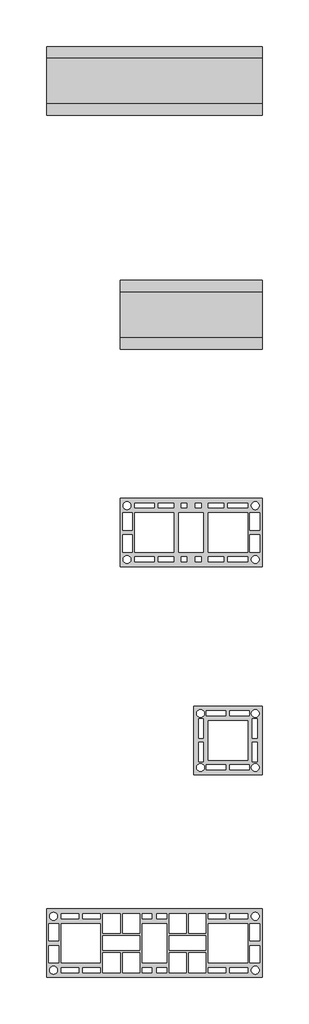
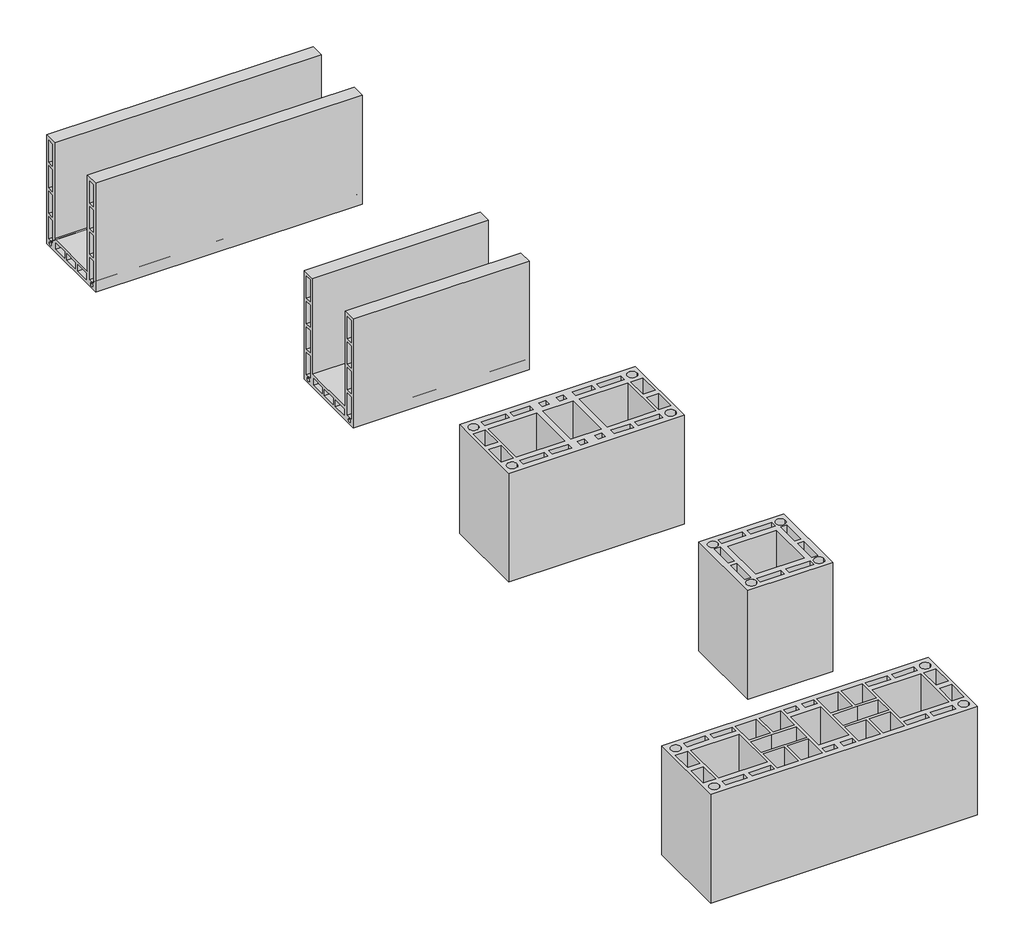
# One storey: 5 proxies.
"""IFC4 building model written with IfcOpenShell, lengths in millimetres."""

import ifcopenshell
import ifcopenshell.guid

model = None  # the IFC model being written
_history = None  # IfcOwnerHistory: only IFC2X3 demands one
_inside = {}  # id of a spatial element -> (the spatial element, [elements in it])
_under = {}  # id of a project, library or spatial element -> (it, [spatial elements below it])
_declared = {}  # id of a project -> (the project, [libraries it declares])
_typed = {}  # id of a type object -> (the type object, [elements of that type])
_made_of = {}  # id of a material, layer set ... -> (it, [elements and type objects made of it])


def new_model(schema):
    """Start an empty IFC model of exactly this schema.

    Asked for "IFC4X3", IfcOpenShell would pick the latest addendum, in which some entities
    have other attributes; the version numbers below select the first issue.
    IFC2X3 requires an IfcOwnerHistory on every rooted entity: one is made here for all.
    """
    global model, _history
    if schema == "IFC4X3":
        model = ifcopenshell.file(schema_version=(4, 3, 0, 0))
    else:
        model = ifcopenshell.file(schema=schema)
    _inside.clear()
    _under.clear()
    _declared.clear()
    _typed.clear()
    _made_of.clear()
    _history = None
    if model.schema == "IFC2X3":
        org = make("IfcOrganization", Name="unknown")
        user = make(
            "IfcPersonAndOrganization",
            ThePerson=make("IfcPerson", FamilyName="unknown"),
            TheOrganization=org,
        )
        app = make(
            "IfcApplication",
            ApplicationDeveloper=org,
            Version="unknown",
            ApplicationFullName="unknown",
            ApplicationIdentifier="unknown",
        )
        _history = make(
            "IfcOwnerHistory",
            OwningUser=user,
            OwningApplication=app,
            ChangeAction="ADDED",
            CreationDate=0,
        )
    return model


def make(cls, **values):
    """One entity of the class cls with the attributes given. An attribute that is None is left unset."""
    return model.create_entity(
        cls, **{name: value for name, value in values.items() if value is not None}
    )


def rooted(cls, **values):
    """An entity with a GlobalId (a new one), such as an element, a storey or a relation."""
    return make(cls, GlobalId=ifcopenshell.guid.new(), OwnerHistory=_history, **values)


def si_unit(unit_type, name, prefix=None):
    """IfcSIUnit, for example si_unit("LENGTHUNIT", "METRE", prefix="MILLI")."""
    return make("IfcSIUnit", UnitType=unit_type, Prefix=prefix, Name=name)


def assignment(units):
    """IfcUnitAssignment: the units of a project."""
    return None if units is None else make("IfcUnitAssignment", Units=units)


def point(xyz):
    """IfcCartesianPoint."""
    return None if xyz is None else make("IfcCartesianPoint", Coordinates=xyz)


def direction(xyz):
    """IfcDirection."""
    return None if xyz is None else make("IfcDirection", DirectionRatios=xyz)


def frame(location, z_axis=None, x_axis=None):
    """IfcAxis2Placement3D, a coordinate frame: its origin and axes. An axis left out is left unset."""
    return make(
        "IfcAxis2Placement3D",
        Location=point(location),
        Axis=direction(z_axis),
        RefDirection=direction(x_axis),
    )


def frame_2d(location, x_axis=None):
    """IfcAxis2Placement2D, a coordinate frame in the plane: its origin and x axis."""
    return make(
        "IfcAxis2Placement2D", Location=point(location), RefDirection=direction(x_axis)
    )


def origin():
    """The frame at (0, 0, 0) with its axes left unset."""
    return frame((0.0, 0.0, 0.0))


def origin_with_axes():
    """The frame at (0, 0, 0) with the z axis (0, 0, 1) and the x axis (1, 0, 0) written out."""
    return frame((0.0, 0.0, 0.0), z_axis=(0.0, 0.0, 1.0), x_axis=(1.0, 0.0, 0.0))


def place(relative_to, where):
    """IfcLocalPlacement: puts the frame where relative to a parent placement (None: the world)."""
    return make(
        "IfcLocalPlacement", PlacementRelTo=relative_to, RelativePlacement=where
    )


def context(
    kind, dimensions, precision=None, world=None, true_north=None, identifier=None
):
    """IfcGeometricRepresentationContext, for example the 3D "Model" context."""
    return make(
        "IfcGeometricRepresentationContext",
        ContextIdentifier=identifier,
        ContextType=kind,
        CoordinateSpaceDimension=dimensions,
        Precision=precision,
        WorldCoordinateSystem=world,
        TrueNorth=true_north,
    )


def project(units=None, contexts=None):
    """IfcProject with its units and contexts."""
    return rooted(
        "IfcProject",
        Name="project",
        RepresentationContexts=contexts,
        UnitsInContext=assignment(units),
    )


def spatial(cls, under=None, at=None, **own):
    """A site, building, storey or space (cls), placed at a placement, below another one or the project."""
    s = rooted(cls, ObjectPlacement=at, **own)
    if under is not None:
        _under.setdefault(under.id(), (under, []))[1].append(s)
    return s


def polyline(points):
    """IfcPolyline through the points."""
    return make("IfcPolyline", Points=[point(p) for p in points])


def circle_curve(where, radius):
    """IfcCircle in the frame where."""
    return make("IfcCircle", Position=where, Radius=radius)


def trimmed(basis, trim1, trim2, sense, master):
    """IfcTrimmedCurve: the piece of a basis curve between two trims."""
    return make(
        "IfcTrimmedCurve",
        BasisCurve=basis,
        Trim1=trim1,
        Trim2=trim2,
        SenseAgreement=sense,
        MasterRepresentation=master,
    )


def segment(curve, same_sense, transition):
    """IfcCompositeCurveSegment."""
    return make(
        "IfcCompositeCurveSegment",
        Transition=transition,
        SameSense=same_sense,
        ParentCurve=curve,
    )


def composite_curve(segments, self_intersect=None):
    """IfcCompositeCurve: segments joined end to end."""
    return make("IfcCompositeCurve", Segments=segments, SelfIntersect=self_intersect)


def outline(outer, holes=None, kind="AREA"):
    """IfcArbitraryClosedProfileDef: a profile drawn as a closed curve; with holes, ...WithVoids."""
    if holes is None:
        return make("IfcArbitraryClosedProfileDef", ProfileType=kind, OuterCurve=outer)
    return make(
        "IfcArbitraryProfileDefWithVoids",
        ProfileType=kind,
        OuterCurve=outer,
        InnerCurves=holes,
    )


def extrude(swept, where, along, depth):
    """IfcExtrudedAreaSolid: the profile swept, set in the frame where, extruded along a direction by depth."""
    return make(
        "IfcExtrudedAreaSolid",
        SweptArea=swept,
        Position=where,
        ExtrudedDirection=direction(along),
        Depth=depth,
    )


def shape(context_of_items, identifier, shape_type, items):
    """IfcShapeRepresentation: the items that make up one representation, for example the "Body"."""
    return make(
        "IfcShapeRepresentation",
        ContextOfItems=context_of_items,
        RepresentationIdentifier=identifier,
        RepresentationType=shape_type,
        Items=items,
    )


def source(mapping_origin, context_of_items, identifier, shape_type, items):
    """IfcRepresentationMap: a shape defined once, which mapped items show again and again."""
    return make(
        "IfcRepresentationMap",
        MappingOrigin=mapping_origin,
        MappedRepresentation=shape(context_of_items, identifier, shape_type, items),
    )


def transform(
    local_origin,
    x_axis=None,
    y_axis=None,
    z_axis=None,
    scale=None,
    scale2=None,
    scale3=None,
    uniform=True,
):
    """IfcCartesianTransformationOperator3D, or its non-uniform kind. x_axis, y_axis, z_axis: its Axis1, 2, 3."""
    if uniform:
        return make(
            "IfcCartesianTransformationOperator3D",
            Axis1=direction(x_axis),
            Axis2=direction(y_axis),
            LocalOrigin=point(local_origin),
            Scale=scale,
            Axis3=direction(z_axis),
        )
    return make(
        "IfcCartesianTransformationOperator3DnonUniform",
        Axis1=direction(x_axis),
        Axis2=direction(y_axis),
        LocalOrigin=point(local_origin),
        Scale=scale,
        Axis3=direction(z_axis),
        Scale2=scale2,
        Scale3=scale3,
    )


def mapped(mapping_source, mapping_target):
    """IfcMappedItem: shows the shape of a source again, moved by a transform."""
    return make(
        "IfcMappedItem", MappingSource=mapping_source, MappingTarget=mapping_target
    )


def made_of(thing, what):
    """Note that an element or type object is made of a material, layer set ...; save() writes the relation."""
    if what is not None:
        _made_of.setdefault(what.id(), (what, []))[1].append(thing)
    return thing


def element(
    cls,
    number,
    at=None,
    inside=None,
    cuts=None,
    type_object=None,
    material=None,
    context=None,
    identifier="Body",
    shape_type=None,
    held_by="IfcProductDefinitionShape",
    body=None,
    shapes=None,
    **own,
):
    """One element of the class cls, such as IfcWall. Its Tag is "e" and its number.

    at: its placement. inside: the storey or other place that contains it. cuts: it is an
    opening in that element (IfcRelVoidsElement). A single representation is given by context,
    identifier, shape_type and body (its items); several are given by shapes. held_by: the class
    of the entity that holds the representations. save() writes the other relations.
    """
    e = rooted(cls, Tag="e%d" % number, ObjectPlacement=at, **own)
    if body is not None:
        shapes = [shape(context, identifier, shape_type, body)]
    if shapes is not None:
        e.Representation = make(held_by, Representations=shapes)
    if inside is not None:
        _inside.setdefault(inside.id(), (inside, []))[1].append(e)
    if cuts is not None:
        rooted(
            "IfcRelVoidsElement", RelatingBuildingElement=cuts, RelatedOpeningElement=e
        )
    if type_object is not None:
        _typed.setdefault(type_object.id(), (type_object, []))[1].append(e)
    return made_of(e, material)


def aggregate(whole, parts):
    """IfcRelAggregates: a whole, such as a stair, and the parts it consists of."""
    return rooted("IfcRelAggregates", RelatingObject=whole, RelatedObjects=parts)


def save(model, path):
    """Write the relations noted so far, then the file.

    IfcRelAggregates (storeys below a building ...), IfcRelContainedInSpatialStructure (elements
    in a storey), IfcRelDefinesByType, IfcRelAssociatesMaterial and IfcRelDeclares: one each for
    every whole, place, type object, material and project.
    """
    for whole, parts in _under.values():
        aggregate(whole, parts)
    for where, things in _inside.values():
        rooted(
            "IfcRelContainedInSpatialStructure",
            RelatedElements=things,
            RelatingStructure=where,
        )
    for kind, things in _typed.values():
        rooted("IfcRelDefinesByType", RelatedObjects=things, RelatingType=kind)
    for what, things in _made_of.values():
        rooted("IfcRelAssociatesMaterial", RelatedObjects=things, RelatingMaterial=what)
    for by, libraries in _declared.values():
        rooted("IfcRelDeclares", RelatingContext=by, RelatedDefinitions=libraries)
    model.write(path)


def bloco_estrutural_de_15cm_l14_be15_329fd50e(model_context):
    return source(origin(), model_context, "Body", "SweptSolid", [
        extrude(outline(polyline([(0.0, 140.0), (140.0, 140.0), (140.0, 0.0), (0.0, 0.0), (0.0, 140.0)]), holes=[polyline([(30.0, 110.0), (30.0, 30.0), (110.0, 30.0), (110.0, 110.0), (30.0, 110.0)]), composite_curve([segment(trimmed(circle_curve(frame_2d((14.1087523, 124.7509514)), 8.0), [point((6.1087523, 124.7509514))], [point((22.1087523, 124.7509514))], True, "CARTESIAN"), True, "CONTINUOUS"), segment(trimmed(circle_curve(frame_2d((14.1087523, 124.7509514)), 8.0), [point((22.1087523, 124.7509514))], [point((6.1087523, 124.7509514))], True, "CARTESIAN"), True, "CONTINUOUS")], self_intersect=False), composite_curve([segment(trimmed(circle_curve(frame_2d((14.1087523, 14.7509514)), 8.0), [point((6.1087523, 14.7509514))], [point((22.1087523, 14.7509514))], True, "CARTESIAN"), True, "CONTINUOUS"), segment(trimmed(circle_curve(frame_2d((14.1087523, 14.7509514)), 8.0), [point((22.1087523, 14.7509514))], [point((6.1087523, 14.7509514))], True, "CARTESIAN"), True, "CONTINUOUS")], self_intersect=False), polyline([(20.0, 66.0), (10.0, 66.0), (10.0, 26.0), (20.0, 26.0), (20.0, 66.0)]), polyline([(20.0, 74.0), (20.0, 114.0), (10.0, 114.0), (10.0, 74.0), (20.0, 74.0)]), composite_curve([segment(trimmed(circle_curve(frame_2d((125.8912477, 124.7509514)), 8.0), [point((133.8912477, 124.7509514))], [point((117.8912477, 124.7509514))], True, "CARTESIAN"), True, "CONTINUOUS"), segment(trimmed(circle_curve(frame_2d((125.8912477, 124.7509514)), 8.0), [point((117.8912477, 124.7509514))], [point((133.8912477, 124.7509514))], True, "CARTESIAN"), True, "CONTINUOUS")], self_intersect=False), composite_curve([segment(trimmed(circle_curve(frame_2d((125.8912477, 14.7509514)), 8.0), [point((133.8912477, 14.7509514))], [point((117.8912477, 14.7509514))], True, "CARTESIAN"), True, "CONTINUOUS"), segment(trimmed(circle_curve(frame_2d((125.8912477, 14.7509514)), 8.0), [point((117.8912477, 14.7509514))], [point((133.8912477, 14.7509514))], True, "CARTESIAN"), True, "CONTINUOUS")], self_intersect=False), polyline([(120.0, 66.0), (120.0, 26.0), (130.0, 26.0), (130.0, 66.0), (120.0, 66.0)]), polyline([(120.0, 74.0), (130.0, 74.0), (130.0, 114.0), (120.0, 114.0), (120.0, 74.0)]), polyline([(66.0, 120.0), (66.0, 130.0), (26.0, 130.0), (26.0, 120.0), (66.0, 120.0)]), polyline([(74.0, 120.0), (114.0, 120.0), (114.0, 130.0), (74.0, 130.0), (74.0, 120.0)]), polyline([(66.0, 20.0), (26.0, 20.0), (26.0, 10.0), (66.0, 10.0), (66.0, 20.0)]), polyline([(74.0, 20.0), (74.0, 10.0), (114.0, 10.0), (114.0, 20.0), (74.0, 20.0)])]), origin_with_axes(), (0.0, 0.0, 1.0), 190.0),
    ])


def bloco_estrutural_de_30cm_l14_be30_19b25b02(model_context):
    return source(origin(), model_context, "Body", "SweptSolid", [
        extrude(outline(polyline([(290.0, 0.0), (0.0, 0.0), (0.0, 140.0), (290.0, 140.0), (290.0, 0.0)]), holes=[composite_curve([segment(trimmed(circle_curve(frame_2d((14.1087523, 124.7509514)), 8.0), [point((6.1087523, 124.7509514))], [point((22.1087523, 124.7509514))], True, "CARTESIAN"), True, "CONTINUOUS"), segment(trimmed(circle_curve(frame_2d((14.1087523, 124.7509514)), 8.0), [point((22.1087523, 124.7509514))], [point((6.1087523, 124.7509514))], True, "CARTESIAN"), True, "CONTINUOUS")], self_intersect=False), composite_curve([segment(trimmed(circle_curve(frame_2d((14.1087523, 14.7509514)), 8.0), [point((6.1087523, 14.7509514))], [point((22.1087523, 14.7509514))], True, "CARTESIAN"), True, "CONTINUOUS"), segment(trimmed(circle_curve(frame_2d((14.1087523, 14.7509514)), 8.0), [point((22.1087523, 14.7509514))], [point((6.1087523, 14.7509514))], True, "CARTESIAN"), True, "CONTINUOUS")], self_intersect=False), polyline([(110.0, 110.0), (30.0, 110.0), (30.0, 30.0), (110.0, 30.0), (110.0, 110.0)]), polyline([(170.0, 110.0), (120.0, 110.0), (120.0, 30.0), (170.0, 30.0), (170.0, 110.0)]), polyline([(70.0, 130.0), (30.0, 130.0), (30.0, 120.0), (70.0, 120.0), (70.0, 130.0)]), polyline([(70.0, 20.0), (30.0, 20.0), (30.0, 10.0), (70.0, 10.0), (70.0, 20.0)]), polyline([(78.0, 130.0), (78.0, 120.0), (110.0, 120.0), (110.0, 130.0), (78.0, 130.0)]), polyline([(78.0, 20.0), (78.0, 10.0), (110.0, 10.0), (110.0, 20.0), (78.0, 20.0)]), composite_curve([segment(trimmed(circle_curve(frame_2d((275.8912477, 124.7509514)), 8.0), [point((283.8912477, 124.7509514))], [point((267.8912477, 124.7509514))], True, "CARTESIAN"), True, "CONTINUOUS"), segment(trimmed(circle_curve(frame_2d((275.8912477, 124.7509514)), 8.0), [point((267.8912477, 124.7509514))], [point((283.8912477, 124.7509514))], True, "CARTESIAN"), True, "CONTINUOUS")], self_intersect=False), composite_curve([segment(trimmed(circle_curve(frame_2d((275.8912477, 14.7509514)), 8.0), [point((283.8912477, 14.7509514))], [point((267.8912477, 14.7509514))], True, "CARTESIAN"), True, "CONTINUOUS"), segment(trimmed(circle_curve(frame_2d((275.8912477, 14.7509514)), 8.0), [point((267.8912477, 14.7509514))], [point((283.8912477, 14.7509514))], True, "CARTESIAN"), True, "CONTINUOUS")], self_intersect=False), polyline([(180.0, 110.0), (180.0, 30.0), (260.0, 30.0), (260.0, 110.0), (180.0, 110.0)]), polyline([(220.0, 130.0), (220.0, 120.0), (260.0, 120.0), (260.0, 130.0), (220.0, 130.0)]), polyline([(220.0, 20.0), (220.0, 10.0), (260.0, 10.0), (260.0, 20.0), (220.0, 20.0)]), polyline([(212.0, 130.0), (180.0, 130.0), (180.0, 120.0), (212.0, 120.0), (212.0, 130.0)]), polyline([(212.0, 20.0), (180.0, 20.0), (180.0, 10.0), (212.0, 10.0), (212.0, 20.0)]), polyline([(25.0, 110.0), (5.0, 110.0), (5.0, 75.0), (25.0, 75.0), (25.0, 110.0)]), polyline([(25.0, 30.0), (25.0, 65.0), (5.0, 65.0), (5.0, 30.0), (25.0, 30.0)]), polyline([(265.0, 110.0), (265.0, 75.0), (285.0, 75.0), (285.0, 110.0), (265.0, 110.0)]), polyline([(265.0, 30.0), (285.0, 30.0), (285.0, 65.0), (265.0, 65.0), (265.0, 30.0)]), polyline([(153.5, 20.0), (153.5, 10.0), (165.5, 10.0), (165.5, 20.0), (153.5, 20.0)]), polyline([(136.5, 20.0), (124.5, 20.0), (124.5, 10.0), (136.5, 10.0), (136.5, 20.0)]), polyline([(153.5, 120.0), (165.5, 120.0), (165.5, 130.0), (153.5, 130.0), (153.5, 120.0)]), polyline([(136.5, 120.0), (136.5, 130.0), (124.5, 130.0), (124.5, 120.0), (136.5, 120.0)])]), origin_with_axes(), (0.0, 0.0, 1.0), 190.0),
    ])


def bloco_estrutural_de_45cm_l14_be45_067f568e(model_context):
    return source(origin(), model_context, "Body", "SweptSolid", [
        extrude(outline(polyline([(440.0, 0.0), (0.0, 0.0), (0.0, 140.0), (440.0, 140.0), (440.0, 0.0)]), holes=[composite_curve([segment(trimmed(circle_curve(frame_2d((14.1087523, 124.7509514)), 8.0), [point((6.1087523, 124.7509514))], [point((22.1087523, 124.7509514))], True, "CARTESIAN"), True, "CONTINUOUS"), segment(trimmed(circle_curve(frame_2d((14.1087523, 124.7509514)), 8.0), [point((22.1087523, 124.7509514))], [point((6.1087523, 124.7509514))], True, "CARTESIAN"), True, "CONTINUOUS")], self_intersect=False), composite_curve([segment(trimmed(circle_curve(frame_2d((14.1087523, 14.7509514)), 8.0), [point((6.1087523, 14.7509514))], [point((22.1087523, 14.7509514))], True, "CARTESIAN"), True, "CONTINUOUS"), segment(trimmed(circle_curve(frame_2d((14.1087523, 14.7509514)), 8.0), [point((22.1087523, 14.7509514))], [point((6.1087523, 14.7509514))], True, "CARTESIAN"), True, "CONTINUOUS")], self_intersect=False), polyline([(110.0, 110.0), (30.0, 110.0), (30.0, 30.0), (110.0, 30.0), (110.0, 110.0)]), polyline([(245.0, 110.0), (195.0, 110.0), (195.0, 30.0), (245.0, 30.0), (245.0, 110.0)]), polyline([(66.0, 130.0), (30.0, 130.0), (30.0, 120.0), (66.0, 120.0), (66.0, 130.0)]), polyline([(66.0, 20.0), (30.0, 20.0), (30.0, 10.0), (66.0, 10.0), (66.0, 20.0)]), polyline([(74.0, 130.0), (74.0, 120.0), (110.0, 120.0), (110.0, 130.0), (74.0, 130.0)]), polyline([(74.0, 20.0), (74.0, 10.0), (110.0, 10.0), (110.0, 20.0), (74.0, 20.0)]), composite_curve([segment(trimmed(circle_curve(frame_2d((425.8912477, 124.7509514)), 8.0), [point((433.8912477, 124.7509514))], [point((417.8912477, 124.7509514))], True, "CARTESIAN"), True, "CONTINUOUS"), segment(trimmed(circle_curve(frame_2d((425.8912477, 124.7509514)), 8.0), [point((417.8912477, 124.7509514))], [point((433.8912477, 124.7509514))], True, "CARTESIAN"), True, "CONTINUOUS")], self_intersect=False), composite_curve([segment(trimmed(circle_curve(frame_2d((425.8912477, 14.7509514)), 8.0), [point((433.8912477, 14.7509514))], [point((417.8912477, 14.7509514))], True, "CARTESIAN"), True, "CONTINUOUS"), segment(trimmed(circle_curve(frame_2d((425.8912477, 14.7509514)), 8.0), [point((417.8912477, 14.7509514))], [point((433.8912477, 14.7509514))], True, "CARTESIAN"), True, "CONTINUOUS")], self_intersect=False), polyline([(330.0, 110.0), (330.0, 30.0), (410.0, 30.0), (410.0, 110.0), (330.0, 110.0)]), polyline([(374.0, 130.0), (374.0, 120.0), (410.0, 120.0), (410.0, 130.0), (374.0, 130.0)]), polyline([(374.0, 20.0), (374.0, 10.0), (410.0, 10.0), (410.0, 20.0), (374.0, 20.0)]), polyline([(366.0, 130.0), (330.0, 130.0), (330.0, 120.0), (366.0, 120.0), (366.0, 130.0)]), polyline([(366.0, 20.0), (330.0, 20.0), (330.0, 10.0), (366.0, 10.0), (366.0, 20.0)]), polyline([(25.0, 110.0), (5.0, 110.0), (5.0, 75.0), (25.0, 75.0), (25.0, 110.0)]), polyline([(25.0, 30.0), (25.0, 65.0), (5.0, 65.0), (5.0, 30.0), (25.0, 30.0)]), polyline([(415.0, 110.0), (415.0, 75.0), (435.0, 75.0), (435.0, 110.0), (415.0, 110.0)]), polyline([(415.0, 30.0), (435.0, 30.0), (435.0, 65.0), (415.0, 65.0), (415.0, 30.0)]), polyline([(225.0, 20.0), (225.0, 10.0), (245.0, 10.0), (245.0, 20.0), (225.0, 20.0)]), polyline([(215.0, 20.0), (195.0, 20.0), (195.0, 10.0), (215.0, 10.0), (215.0, 20.0)]), polyline([(225.0, 120.0), (245.0, 120.0), (245.0, 130.0), (225.0, 130.0), (225.0, 120.0)]), polyline([(215.0, 120.0), (215.0, 130.0), (195.0, 130.0), (195.0, 120.0), (215.0, 120.0)]), polyline([(150.0, 130.0), (115.0, 130.0), (115.0, 90.0), (150.0, 90.0), (150.0, 130.0)]), polyline([(190.0, 130.0), (155.0, 130.0), (155.0, 90.0), (190.0, 90.0), (190.0, 130.0)]), polyline([(115.0, 85.0), (115.0, 55.0), (190.0, 55.0), (190.0, 85.0), (148.9828076, 85.0), (115.0, 85.0)]), polyline([(155.0, 50.0), (155.0, 10.0), (190.0, 10.0), (190.0, 50.0), (155.0, 50.0)]), polyline([(150.0, 10.0), (150.0, 50.0), (115.0, 50.0), (115.0, 10.0), (150.0, 10.0)]), polyline([(290.0, 130.0), (290.0, 90.0), (325.0, 90.0), (325.0, 130.0), (290.0, 130.0)]), polyline([(250.0, 130.0), (250.0, 90.0), (285.0, 90.0), (285.0, 130.0), (250.0, 130.0)]), polyline([(325.0, 85.0), (291.0171924, 85.0), (250.0, 85.0), (250.0, 55.0), (291.0171924, 55.0), (325.0, 55.0), (325.0, 85.0)]), polyline([(285.0, 50.0), (250.0, 50.0), (250.0, 10.0), (285.0, 10.0), (285.0, 50.0)]), polyline([(290.0, 10.0), (325.0, 10.0), (325.0, 50.0), (290.0, 50.0), (290.0, 10.0)])]), origin_with_axes(), (0.0, 0.0, 1.0), 190.0),
    ])


def canaleta_l14_c30_6f9dc855(model_context):
    return source(origin(), model_context, "Body", "SweptSolid", [
        extrude(outline(polyline([(140.0, 0.0), (0.0, 0.0), (0.0, 190.0), (23.0, 190.0), (23.0, 23.0), (117.0, 23.0), (117.0, 190.0), (140.0, 190.0), (140.0, 0.0)]), holes=[polyline([(123.0, 184.0), (123.0, 145.5), (134.0, 145.5), (134.0, 184.0), (123.0, 184.0)]), polyline([(123.0, 139.5), (123.0, 101.0), (134.0, 101.0), (134.0, 139.5), (123.0, 139.5)]), polyline([(123.0, 95.0), (123.0, 56.5), (134.0, 56.5), (134.0, 95.0), (123.0, 95.0)]), polyline([(123.0, 50.5), (123.0, 12.0), (134.0, 12.0), (134.0, 50.5), (123.0, 50.5)]), composite_curve([segment(trimmed(circle_curve(frame_2d((128.9426557, 6.2112346)), 3.0), [point((125.9426557, 6.2112346))], [point((131.9426557, 6.2112346))], True, "CARTESIAN"), True, "CONTINUOUS"), segment(trimmed(circle_curve(frame_2d((128.9426557, 6.2112346)), 3.0), [point((131.9426557, 6.2112346))], [point((125.9426557, 6.2112346))], True, "CARTESIAN"), True, "CONTINUOUS")], self_intersect=False), polyline([(17.0, 184.0), (6.0, 184.0), (6.0, 145.5), (17.0, 145.5), (17.0, 184.0)]), polyline([(17.0, 139.5), (6.0, 139.5), (6.0, 101.0), (17.0, 101.0), (17.0, 139.5)]), polyline([(17.0, 95.0), (6.0, 95.0), (6.0, 56.5), (17.0, 56.5), (17.0, 95.0)]), polyline([(17.0, 50.5), (6.0, 50.5), (6.0, 12.0), (17.0, 12.0), (17.0, 50.5)]), composite_curve([segment(trimmed(circle_curve(frame_2d((11.0573443, 6.2112346)), 3.0), [point((8.0573443, 6.2112346))], [point((14.0573443, 6.2112346))], True, "CARTESIAN"), True, "CONTINUOUS"), segment(trimmed(circle_curve(frame_2d((11.0573443, 6.2112346)), 3.0), [point((14.0573443, 6.2112346))], [point((8.0573443, 6.2112346))], True, "CARTESIAN"), True, "CONTINUOUS")], self_intersect=False), polyline([(88.5, 17.0), (88.5, 6.0), (113.5, 6.0), (113.5, 17.0), (88.5, 17.0)]), polyline([(57.5, 17.0), (57.5, 6.0), (82.5, 6.0), (82.5, 17.0), (57.5, 17.0)]), polyline([(26.5, 17.0), (26.5, 6.0), (51.5, 6.0), (51.5, 17.0), (26.5, 17.0)])]), frame((0.0, 0.0, 0.0), z_axis=(1.0, 0.0, 0.0), x_axis=(0.0, 1.0, 0.0)), (0.0, 0.0, 1.0), 290.0),
    ])


def canaleta_l14_c45_c2fd00c5(model_context):
    return source(origin(), model_context, "Body", "SweptSolid", [
        extrude(outline(polyline([(140.0, 0.0), (0.0, 0.0), (0.0, 190.0), (23.0, 190.0), (23.0, 23.0), (117.0, 23.0), (117.0, 190.0), (140.0, 190.0), (140.0, 0.0)]), holes=[polyline([(123.0, 184.0), (123.0, 145.5), (134.0, 145.5), (134.0, 184.0), (123.0, 184.0)]), polyline([(123.0, 139.5), (123.0, 101.0), (134.0, 101.0), (134.0, 139.5), (123.0, 139.5)]), polyline([(123.0, 95.0), (123.0, 56.5), (134.0, 56.5), (134.0, 95.0), (123.0, 95.0)]), polyline([(123.0, 50.5), (123.0, 12.0), (134.0, 12.0), (134.0, 50.5), (123.0, 50.5)]), composite_curve([segment(trimmed(circle_curve(frame_2d((128.9426557, 6.2112346)), 3.0), [point((125.9426557, 6.2112346))], [point((131.9426557, 6.2112346))], True, "CARTESIAN"), True, "CONTINUOUS"), segment(trimmed(circle_curve(frame_2d((128.9426557, 6.2112346)), 3.0), [point((131.9426557, 6.2112346))], [point((125.9426557, 6.2112346))], True, "CARTESIAN"), True, "CONTINUOUS")], self_intersect=False), polyline([(17.0, 184.0), (6.0, 184.0), (6.0, 145.5), (17.0, 145.5), (17.0, 184.0)]), polyline([(17.0, 139.5), (6.0, 139.5), (6.0, 101.0), (17.0, 101.0), (17.0, 139.5)]), polyline([(17.0, 95.0), (6.0, 95.0), (6.0, 56.5), (17.0, 56.5), (17.0, 95.0)]), polyline([(17.0, 50.5), (6.0, 50.5), (6.0, 12.0), (17.0, 12.0), (17.0, 50.5)]), composite_curve([segment(trimmed(circle_curve(frame_2d((11.0573443, 6.2112346)), 3.0), [point((8.0573443, 6.2112346))], [point((14.0573443, 6.2112346))], True, "CARTESIAN"), True, "CONTINUOUS"), segment(trimmed(circle_curve(frame_2d((11.0573443, 6.2112346)), 3.0), [point((14.0573443, 6.2112346))], [point((8.0573443, 6.2112346))], True, "CARTESIAN"), True, "CONTINUOUS")], self_intersect=False), polyline([(88.5, 17.0), (88.5, 6.0), (113.5, 6.0), (113.5, 17.0), (88.5, 17.0)]), polyline([(57.5, 17.0), (57.5, 6.0), (82.5, 6.0), (82.5, 17.0), (57.5, 17.0)]), polyline([(26.5, 17.0), (26.5, 6.0), (51.5, 6.0), (51.5, 17.0), (26.5, 17.0)])]), frame((0.0, 0.0, 0.0), z_axis=(1.0, 0.0, 0.0), x_axis=(0.0, 1.0, 0.0)), (0.0, 0.0, 1.0), 440.0),
    ])


model = new_model("IFC4")

# Units and contexts
model_context = context("Model", 3, world=origin())
ifc_project = project(units=[si_unit("LENGTHUNIT", "METRE", prefix="MILLI")], contexts=[model_context])

# Site, building, storey
site = spatial("IfcSite", under=ifc_project)
building = spatial("IfcBuilding", under=site)
storey = spatial("IfcBuildingStorey", under=building, Name="Nível 1", Elevation=0.0)

# Proxies
placement = place(None, origin())
bloco_estrutural_de_15cm_l14_be15_shape = bloco_estrutural_de_15cm_l14_be15_329fd50e(model_context)
element("IfcBuildingElementProxy", 1, Name="Bloco Estrutural de 15cm (L14) : BE15", ObjectType="Bloco Estrutural de 15cm (L14) : BE15", at=placement, inside=storey, context=model_context, shape_type="MappedRepresentation", body=[
    mapped(bloco_estrutural_de_15cm_l14_be15_shape, transform((2691.9297154, 1590.0313854, 0.0), x_axis=(1.0, 0.0, 0.0), y_axis=(0.0, 1.0, 0.0), z_axis=(0.0, 0.0, 1.0))),
])
bloco_estrutural_de_30cm_l14_be30_shape = bloco_estrutural_de_30cm_l14_be30_19b25b02(model_context)
element("IfcBuildingElementProxy", 2, Name="Bloco Estrutural de 30cm (L14) : BE30", ObjectType="Bloco Estrutural de 30cm (L14) : BE30", at=placement, inside=storey, context=model_context, shape_type="MappedRepresentation", body=[
    mapped(bloco_estrutural_de_30cm_l14_be30_shape, transform((2541.9297154, 2014.2243668, 0.0), x_axis=(1.0, 0.0, 0.0), y_axis=(0.0, 1.0, 0.0), z_axis=(0.0, 0.0, 1.0))),
])
bloco_estrutural_de_45cm_l14_be45_shape = bloco_estrutural_de_45cm_l14_be45_067f568e(model_context)
element("IfcBuildingElementProxy", 3, Name="Bloco Estrutural de 45cm (L14) : BE45", ObjectType="Bloco Estrutural de 45cm (L14) : BE45", at=placement, inside=storey, context=model_context, shape_type="MappedRepresentation", body=[
    mapped(bloco_estrutural_de_45cm_l14_be45_shape, transform((2391.9297154, 1176.4687225, 0.0), x_axis=(1.0, 0.0, 0.0), y_axis=(0.0, 1.0, 0.0), z_axis=(0.0, 0.0, 1.0))),
])
canaleta_l14_c30_shape = canaleta_l14_c30_6f9dc855(model_context)
element("IfcBuildingElementProxy", 4, Name="Canaleta (L14) : C30", ObjectType="Canaleta (L14) : C30", at=placement, inside=storey, context=model_context, shape_type="MappedRepresentation", body=[
    mapped(canaleta_l14_c30_shape, transform((2541.9297154, 2458.4083893, 0.0), x_axis=(1.0, 0.0, 0.0), y_axis=(0.0, 1.0, 0.0), z_axis=(0.0, 0.0, 1.0))),
])
canaleta_l14_c45_shape = canaleta_l14_c45_c2fd00c5(model_context)
element("IfcBuildingElementProxy", 5, Name="Canaleta (L14) : C45", ObjectType="Canaleta (L14) : C45", at=placement, inside=storey, context=model_context, shape_type="MappedRepresentation", body=[
    mapped(canaleta_l14_c45_shape, transform((2391.9297154, 2935.4953738, 0.0), x_axis=(1.0, 0.0, 0.0), y_axis=(0.0, 1.0, 0.0), z_axis=(0.0, 0.0, 1.0))),
])

save(model, "model.ifc")

# Revit data of these elements
# Project information
#   Data de emissão do projeto = "Data de emissão"
#   Status do projeto = "Status do projeto"
#   Nome do cliente = "Proprietário"
#   Endereço do projeto = "Enter address here"
#   Nome do projeto = "Nome do projeto"
#   Número do projeto = "0001"
# Type "Bloco Estrutural de 15cm (L14) : BE15"
#   Material [instance default] = Blocos Cerâmicos
# Type "Bloco Estrutural de 30cm (L14) : BE30"
#   Material [instance default] = Blocos Cerâmicos
# Type "Bloco Estrutural de 45cm (L14) : BE45"
#   Material [instance default] = Blocos Cerâmicos
# Type "Canaleta (L14) : C30"
#   Comprimento = 290 mm
#   Material [instance default] = Blocos Cerâmicos
# Type "Canaleta (L14) : C45"
#   Comprimento = 440 mm
#   Material [instance default] = Blocos Cerâmicos
# Element 1 (IfcBuildingElementProxy, "Bloco Estrutural de 15cm (L14) : BE15")
#   Material = Blocos Cerâmicos
#   Phase Created = Construção nova
#   Materials on its faces: "Blocos Cerâmicos"
# Element 2 (IfcBuildingElementProxy, "Bloco Estrutural de 30cm (L14) : BE30")
#   Material = Blocos Cerâmicos
#   Phase Created = Construção nova
#   Materials on its faces: "Blocos Cerâmicos"
# Element 3 (IfcBuildingElementProxy, "Bloco Estrutural de 45cm (L14) : BE45")
#   Material = Blocos Cerâmicos
#   Phase Created = Construção nova
#   Materials on its faces: "Blocos Cerâmicos"
# Element 4 (IfcBuildingElementProxy, "Canaleta (L14) : C30")
#   Material = Blocos Cerâmicos
#   Phase Created = Construção nova
#   Materials on its faces: "Blocos Cerâmicos"
# Element 5 (IfcBuildingElementProxy, "Canaleta (L14) : C45")
#   Material = Blocos Cerâmicos
#   Phase Created = Construção nova
#   Materials on its faces: "Blocos Cerâmicos"
# Materials
#   "Blocos Cerâmicos": class "Genérico", colour RGB 120 120 120, transparency 0, Cost = 0
